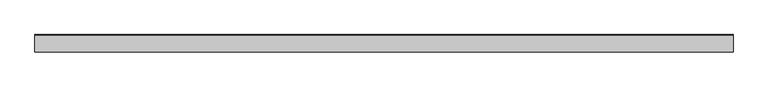
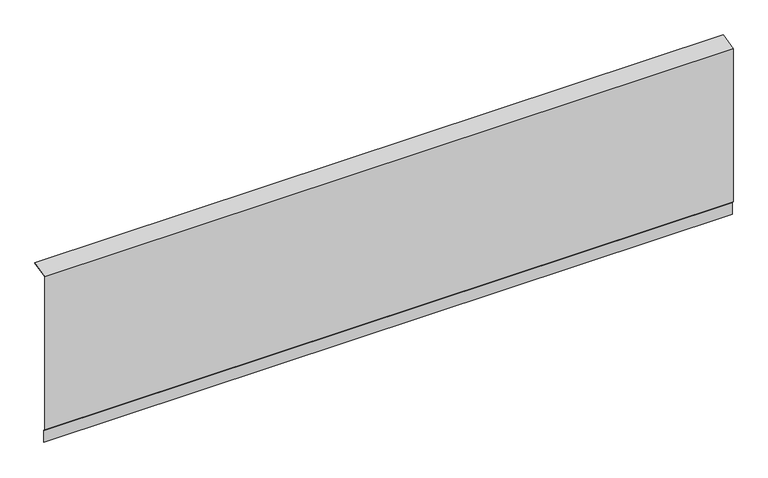
"""IFC4 building model written with IfcOpenShell, lengths in millimetres: proxy geometry, Membrane002 1149 : Membrane002 1149."""

import ifcopenshell
import ifcopenshell.guid

model = None  # the IFC model being written
_history = None  # IfcOwnerHistory: only IFC2X3 demands one
_inside = {}  # id of a spatial element -> (the spatial element, [elements in it])
_under = {}  # id of a project, library or spatial element -> (it, [spatial elements below it])
_declared = {}  # id of a project -> (the project, [libraries it declares])
_typed = {}  # id of a type object -> (the type object, [elements of that type])
_made_of = {}  # id of a material, layer set ... -> (it, [elements and type objects made of it])


def new_model(schema):
    """Start an empty IFC model of exactly this schema.

    Asked for "IFC4X3", IfcOpenShell would pick the latest addendum, in which some entities
    have other attributes; the version numbers below select the first issue.
    IFC2X3 requires an IfcOwnerHistory on every rooted entity: one is made here for all.
    """
    global model, _history
    if schema == "IFC4X3":
        model = ifcopenshell.file(schema_version=(4, 3, 0, 0))
    else:
        model = ifcopenshell.file(schema=schema)
    _inside.clear()
    _under.clear()
    _declared.clear()
    _typed.clear()
    _made_of.clear()
    _history = None
    if model.schema == "IFC2X3":
        org = make("IfcOrganization", Name="unknown")
        user = make(
            "IfcPersonAndOrganization",
            ThePerson=make("IfcPerson", FamilyName="unknown"),
            TheOrganization=org,
        )
        app = make(
            "IfcApplication",
            ApplicationDeveloper=org,
            Version="unknown",
            ApplicationFullName="unknown",
            ApplicationIdentifier="unknown",
        )
        _history = make(
            "IfcOwnerHistory",
            OwningUser=user,
            OwningApplication=app,
            ChangeAction="ADDED",
            CreationDate=0,
        )
    return model


def make(cls, **values):
    """One entity of the class cls with the attributes given. An attribute that is None is left unset."""
    return model.create_entity(
        cls, **{name: value for name, value in values.items() if value is not None}
    )


def rooted(cls, **values):
    """An entity with a GlobalId (a new one), such as an element, a storey or a relation."""
    return make(cls, GlobalId=ifcopenshell.guid.new(), OwnerHistory=_history, **values)


def si_unit(unit_type, name, prefix=None):
    """IfcSIUnit, for example si_unit("LENGTHUNIT", "METRE", prefix="MILLI")."""
    return make("IfcSIUnit", UnitType=unit_type, Prefix=prefix, Name=name)


def assignment(units):
    """IfcUnitAssignment: the units of a project."""
    return None if units is None else make("IfcUnitAssignment", Units=units)


def point(xyz):
    """IfcCartesianPoint."""
    return None if xyz is None else make("IfcCartesianPoint", Coordinates=xyz)


def direction(xyz):
    """IfcDirection."""
    return None if xyz is None else make("IfcDirection", DirectionRatios=xyz)


def frame(location, z_axis=None, x_axis=None):
    """IfcAxis2Placement3D, a coordinate frame: its origin and axes. An axis left out is left unset."""
    return make(
        "IfcAxis2Placement3D",
        Location=point(location),
        Axis=direction(z_axis),
        RefDirection=direction(x_axis),
    )


def origin():
    """The frame at (0, 0, 0) with its axes left unset."""
    return frame((0.0, 0.0, 0.0))


def place(relative_to, where):
    """IfcLocalPlacement: puts the frame where relative to a parent placement (None: the world)."""
    return make(
        "IfcLocalPlacement", PlacementRelTo=relative_to, RelativePlacement=where
    )


def context(
    kind, dimensions, precision=None, world=None, true_north=None, identifier=None
):
    """IfcGeometricRepresentationContext, for example the 3D "Model" context."""
    return make(
        "IfcGeometricRepresentationContext",
        ContextIdentifier=identifier,
        ContextType=kind,
        CoordinateSpaceDimension=dimensions,
        Precision=precision,
        WorldCoordinateSystem=world,
        TrueNorth=true_north,
    )


def project(units=None, contexts=None):
    """IfcProject with its units and contexts."""
    return rooted(
        "IfcProject",
        Name="project",
        RepresentationContexts=contexts,
        UnitsInContext=assignment(units),
    )


def spatial(cls, under=None, at=None, **own):
    """A site, building, storey or space (cls), placed at a placement, below another one or the project."""
    s = rooted(cls, ObjectPlacement=at, **own)
    if under is not None:
        _under.setdefault(under.id(), (under, []))[1].append(s)
    return s


def polyline(points):
    """IfcPolyline through the points."""
    return make("IfcPolyline", Points=[point(p) for p in points])


def outline(outer, holes=None, kind="AREA"):
    """IfcArbitraryClosedProfileDef: a profile drawn as a closed curve; with holes, ...WithVoids."""
    if holes is None:
        return make("IfcArbitraryClosedProfileDef", ProfileType=kind, OuterCurve=outer)
    return make(
        "IfcArbitraryProfileDefWithVoids",
        ProfileType=kind,
        OuterCurve=outer,
        InnerCurves=holes,
    )


def extrude(swept, where, along, depth):
    """IfcExtrudedAreaSolid: the profile swept, set in the frame where, extruded along a direction by depth."""
    return make(
        "IfcExtrudedAreaSolid",
        SweptArea=swept,
        Position=where,
        ExtrudedDirection=direction(along),
        Depth=depth,
    )


def shape(context_of_items, identifier, shape_type, items):
    """IfcShapeRepresentation: the items that make up one representation, for example the "Body"."""
    return make(
        "IfcShapeRepresentation",
        ContextOfItems=context_of_items,
        RepresentationIdentifier=identifier,
        RepresentationType=shape_type,
        Items=items,
    )


def source(mapping_origin, context_of_items, identifier, shape_type, items):
    """IfcRepresentationMap: a shape defined once, which mapped items show again and again."""
    return make(
        "IfcRepresentationMap",
        MappingOrigin=mapping_origin,
        MappedRepresentation=shape(context_of_items, identifier, shape_type, items),
    )


def transform(
    local_origin,
    x_axis=None,
    y_axis=None,
    z_axis=None,
    scale=None,
    scale2=None,
    scale3=None,
    uniform=True,
):
    """IfcCartesianTransformationOperator3D, or its non-uniform kind. x_axis, y_axis, z_axis: its Axis1, 2, 3."""
    if uniform:
        return make(
            "IfcCartesianTransformationOperator3D",
            Axis1=direction(x_axis),
            Axis2=direction(y_axis),
            LocalOrigin=point(local_origin),
            Scale=scale,
            Axis3=direction(z_axis),
        )
    return make(
        "IfcCartesianTransformationOperator3DnonUniform",
        Axis1=direction(x_axis),
        Axis2=direction(y_axis),
        LocalOrigin=point(local_origin),
        Scale=scale,
        Axis3=direction(z_axis),
        Scale2=scale2,
        Scale3=scale3,
    )


def mapped(mapping_source, mapping_target):
    """IfcMappedItem: shows the shape of a source again, moved by a transform."""
    return make(
        "IfcMappedItem", MappingSource=mapping_source, MappingTarget=mapping_target
    )


def made_of(thing, what):
    """Note that an element or type object is made of a material, layer set ...; save() writes the relation."""
    if what is not None:
        _made_of.setdefault(what.id(), (what, []))[1].append(thing)
    return thing


def element(
    cls,
    number,
    at=None,
    inside=None,
    cuts=None,
    type_object=None,
    material=None,
    context=None,
    identifier="Body",
    shape_type=None,
    held_by="IfcProductDefinitionShape",
    body=None,
    shapes=None,
    **own,
):
    """One element of the class cls, such as IfcWall. Its Tag is "e" and its number.

    at: its placement. inside: the storey or other place that contains it. cuts: it is an
    opening in that element (IfcRelVoidsElement). A single representation is given by context,
    identifier, shape_type and body (its items); several are given by shapes. held_by: the class
    of the entity that holds the representations. save() writes the other relations.
    """
    e = rooted(cls, Tag="e%d" % number, ObjectPlacement=at, **own)
    if body is not None:
        shapes = [shape(context, identifier, shape_type, body)]
    if shapes is not None:
        e.Representation = make(held_by, Representations=shapes)
    if inside is not None:
        _inside.setdefault(inside.id(), (inside, []))[1].append(e)
    if cuts is not None:
        rooted(
            "IfcRelVoidsElement", RelatingBuildingElement=cuts, RelatedOpeningElement=e
        )
    if type_object is not None:
        _typed.setdefault(type_object.id(), (type_object, []))[1].append(e)
    return made_of(e, material)


def aggregate(whole, parts):
    """IfcRelAggregates: a whole, such as a stair, and the parts it consists of."""
    return rooted("IfcRelAggregates", RelatingObject=whole, RelatedObjects=parts)


def save(model, path):
    """Write the relations noted so far, then the file.

    IfcRelAggregates (storeys below a building ...), IfcRelContainedInSpatialStructure (elements
    in a storey), IfcRelDefinesByType, IfcRelAssociatesMaterial and IfcRelDeclares: one each for
    every whole, place, type object, material and project.
    """
    for whole, parts in _under.values():
        aggregate(whole, parts)
    for where, things in _inside.values():
        rooted(
            "IfcRelContainedInSpatialStructure",
            RelatedElements=things,
            RelatingStructure=where,
        )
    for kind, things in _typed.values():
        rooted("IfcRelDefinesByType", RelatedObjects=things, RelatingType=kind)
    for what, things in _made_of.values():
        rooted("IfcRelAssociatesMaterial", RelatedObjects=things, RelatingMaterial=what)
    for by, libraries in _declared.values():
        rooted("IfcRelDeclares", RelatingContext=by, RelatedDefinitions=libraries)
    model.write(path)


def generic_models_9e557cb2(model_context):
    return source(origin(), model_context, "Body", "SweptSolid", [
        extrude(outline(polyline([(10487.9371885, 43422.3848589), (10439.3258229, 43410.2922698), (10439.3258229, 42942.4837007), (10444.2086354, 42936.2102632), (10444.2086354, 42900.5039063), (10442.7086354, 42900.5039063), (10442.7086354, 42935.6953125), (10437.8258229, 42941.96875), (10437.8258229, 43411.4648438), (10487.5750834, 43423.8404962), (10487.9371885, 43422.3848589)])), frame((3694.2883192, 0.0, 0.0), z_axis=(1.0, 0.0, 0.0), x_axis=(0.0, 1.0, 0.0)), (0.0, 0.0, 1.0), 2000.0),
    ])


if __name__ == "__main__":
    model = new_model("IFC4")
    model_context = context("Model", 3, world=origin())
    ifc_project = project(units=[si_unit("LENGTHUNIT", "METRE", prefix="MILLI")], contexts=[model_context])
    site = spatial("IfcSite", under=ifc_project)
    building = spatial("IfcBuilding", under=site)
    placement = place(None, origin())
    generic_models_shape = generic_models_9e557cb2(model_context)
    element("IfcBuildingElementProxy", 1, Name="Membrane002 1149 : Membrane002 1149", ObjectType="Membrane002 1149 : Membrane002 1149", at=placement, inside=building, context=model_context, shape_type="MappedRepresentation", body=[
        mapped(generic_models_shape, transform((0.0, 0.0, 0.0), x_axis=(1.0, 0.0, 0.0), y_axis=(0.0, 1.0, 0.0), z_axis=(0.0, 0.0, 1.0))),
    ])
    save(model, "model.ifc")

# Revit data of these elements
# Type "Membrane002 1149 : Membrane002 1149"
#   NameOverride = "Membrane002"
# Element 1 (IfcBuildingElementProxy, "Membrane002 1149 : Membrane002 1149")
#   Materials on its faces: "2 LAYERS NO. 30 ASTM D226 ASPHALT SATURATED ORGANIC FELT"
# Materials
#   "2 LAYERS NO. 30 ASTM D226 ASPHALT SATURATED ORGANIC FELT": class "Unassigned", colour RGB 46 171 0, transparency 0
